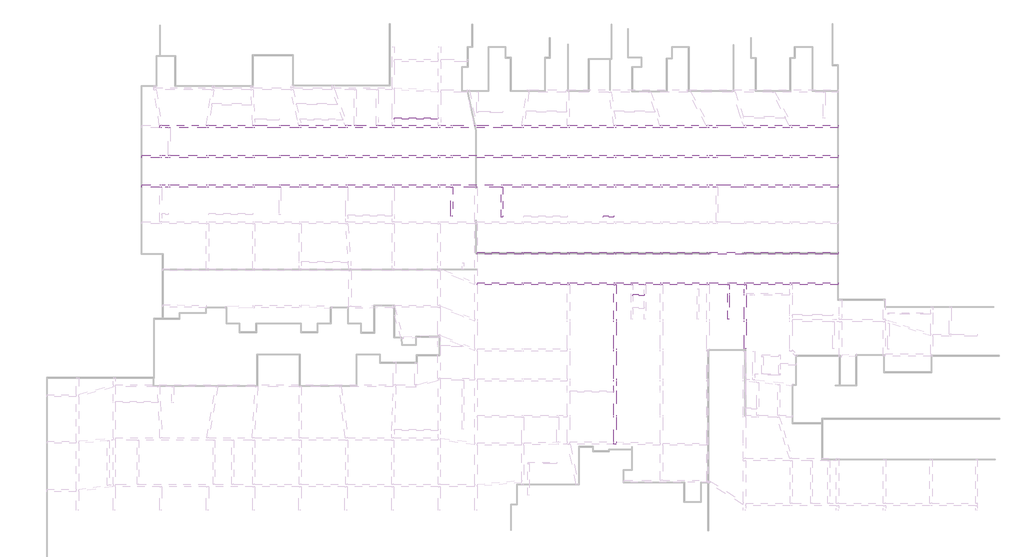
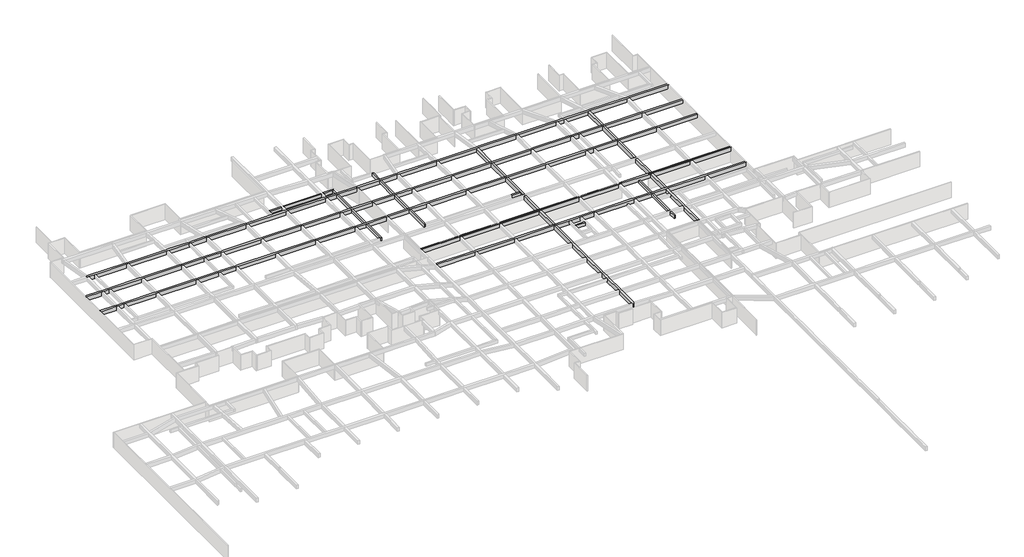
# One storey, part 15 of 16: 13 beams.
"""IFC4 building model written with IfcOpenShell, lengths in millimetres."""

from ifc_helpers import new_model, si_unit, frame, origin, place, context, project, spatial, polyline, outline, extrude, faceted_brep, element, save

model = new_model("IFC4")

# Units and contexts
model_context = context("Model", 3, world=origin())
ifc_project = project(units=[si_unit("LENGTHUNIT", "METRE", prefix="MILLI")], contexts=[model_context])

# Site, building, storey
site = spatial("IfcSite", under=ifc_project)
building = spatial("IfcBuilding", under=site)
storey = spatial("IfcBuildingStorey", under=building, Name="户型图", Elevation=0.0)

# Beams
placement = place(None, origin())
element("IfcBeam", 1, ObjectType="混凝土 - 矩形梁 : KL_beam", at=placement, inside=storey, context=model_context, shape_type="Brep", body=[
    faceted_brep([(204626.3581141, 190295.7397162, 3300.0), (204626.3581141, 189895.7397162, 3300.0), (204626.3581141, 189895.7397162, 2500.0), (204626.3581141, 190295.7397162, 2500.0), (196548.907663, 190295.7397162, 3300.0), (196099.6244537, 190295.7397162, 3300.0), (188560.8339464, 190295.7397162, 3300.0), (188139.6298053, 190295.7397162, 3300.0), (183653.5662503, 190295.7397162, 3300.0), (183353.5662503, 190295.7397162, 3300.0), (182035.6002826, 190295.7397162, 3300.0), (181581.1727256, 190295.7397162, 3300.0), (173958.7712722, 190295.7397162, 3300.0), (173535.6280152, 190295.7397162, 3300.0), (165889.741752, 190295.7397162, 3300.0), (165485.7043374, 190295.7397162, 3300.0), (157809.3486586, 190295.7397162, 3300.0), (157409.1048409, 190295.7397162, 3300.0), (149847.7648646, 190295.7397162, 3300.0), (149443.4649924, 190295.7397162, 3300.0), (146146.1090193, 190295.7397162, 3300.0), (145846.1090193, 190295.7397162, 3300.0), (141582.1467117, 190295.7397162, 3300.0), (141173.2104737, 190295.7397162, 3300.0), (137401.0841862, 190295.7397162, 3300.0), (137101.0841862, 190295.7397162, 3300.0), (135274.2374796, 190295.7397162, 3300.0), (134874.2374796, 190295.7397162, 3300.0), (127216.2109037, 190295.7397162, 3300.0), (126816.2109037, 190295.7397162, 3300.0), (124373.9303911, 190295.7397162, 3300.0), (124073.9303911, 190295.7397162, 3300.0), (120573.9609037, 190295.7397162, 3300.0), (120273.9609037, 190295.7397162, 3300.0), (119056.2524113, 190295.7397162, 3300.0), (118630.5813023, 190295.7397162, 3300.0), (110975.298087, 190295.7397162, 3300.0), (110564.7764439, 190295.7397162, 3300.0), (107420.783903, 190295.7397162, 3300.0), (107120.783903, 190295.7397162, 3300.0), (102906.003817, 190295.7397162, 3300.0), (102505.4548786, 190295.7397162, 3300.0), (94846.2845851, 190295.7397162, 3300.0), (94442.3535561, 190295.7397162, 3300.0), (86664.9777116, 190295.7397162, 3300.0), (86294.1615746, 190295.7397162, 3300.0), (86294.1615746, 189895.7397162, 3300.0), (86694.1615746, 189895.7397162, 3300.0), (87820.783903, 189895.7397162, 3300.0), (88120.783903, 189895.7397162, 3300.0), (94416.2109037, 189895.7397162, 3300.0), (94816.2109037, 189895.7397162, 3300.0), (102516.2109037, 189895.7397162, 3300.0), (102916.2109037, 189895.7397162, 3300.0), (107120.783903, 189895.7397162, 3300.0), (107420.783903, 189895.7397162, 3300.0), (110616.2109037, 189895.7397162, 3300.0), (111016.2109037, 189895.7397162, 3300.0), (118716.2109037, 189895.7397162, 3300.0), (119116.2109037, 189895.7397162, 3300.0), (126816.2109037, 189895.7397162, 3300.0), (127216.2109037, 189895.7397162, 3300.0), (134816.2109037, 189895.7397162, 3300.0), (135216.2109037, 189895.7397162, 3300.0), (137101.0841862, 189895.7397162, 3300.0), (137401.0841862, 189895.7397162, 3300.0), (145846.1090193, 189895.7397162, 3300.0), (146146.1090193, 189895.7397162, 3300.0), (149416.2109037, 189895.7397162, 3300.0), (149816.2109037, 189895.7397162, 3300.0), (157416.2109037, 189895.7397162, 3300.0), (157816.2109037, 189895.7397162, 3300.0), (165516.2109037, 189895.7397162, 3300.0), (165916.2109037, 189895.7397162, 3300.0), (173616.2109037, 189895.7397162, 3300.0), (174016.2109037, 189895.7397162, 3300.0), (181716.2109037, 189895.7397162, 3300.0), (182116.2109037, 189895.7397162, 3300.0), (183353.5662503, 189895.7397162, 3300.0), (183653.5662503, 189895.7397162, 3300.0), (188216.2109037, 189895.7397162, 3300.0), (188616.2109037, 189895.7397162, 3300.0), (196226.5590225, 189895.7397162, 3300.0), (196626.5590225, 189895.7397162, 3300.0), (86294.1615746, 189895.7397162, 2500.0), (86694.1615746, 189895.7397162, 2500.0), (94416.2109037, 189895.7397162, 2500.0), (94816.2109037, 189895.7397162, 2500.0), (102516.2109037, 189895.7397162, 2500.0), (102916.2109037, 189895.7397162, 2500.0), (110616.2109037, 189895.7397162, 2500.0), (111016.2109037, 189895.7397162, 2500.0), (118716.2109037, 189895.7397162, 2500.0), (119116.2109037, 189895.7397162, 2500.0), (126816.2109037, 189895.7397162, 2500.0), (127216.2109037, 189895.7397162, 2500.0), (134816.2109037, 189895.7397162, 2500.0), (135216.2109037, 189895.7397162, 2500.0), (149416.2109037, 189895.7397162, 2500.0), (149816.2109037, 189895.7397162, 2500.0), (157416.2109037, 189895.7397162, 2500.0), (157816.2109037, 189895.7397162, 2500.0), (165516.2109037, 189895.7397162, 2500.0), (165916.2109037, 189895.7397162, 2500.0), (173616.2109037, 189895.7397162, 2500.0), (174016.2109037, 189895.7397162, 2500.0), (181716.2109037, 189895.7397162, 2500.0), (182116.2109037, 189895.7397162, 2500.0), (188216.2109037, 189895.7397162, 2500.0), (188616.2109037, 189895.7397162, 2500.0), (196226.5590225, 189895.7397162, 2500.0), (196626.5590225, 189895.7397162, 2500.0), (86294.1615746, 190295.7397162, 2500.0), (86664.9777116, 190295.7397162, 2500.0), (94442.3535561, 190295.7397162, 2500.0), (94846.2845851, 190295.7397162, 2500.0), (102505.4548786, 190295.7397162, 2500.0), (102906.003817, 190295.7397162, 2500.0), (110564.7764439, 190295.7397162, 2500.0), (110975.298087, 190295.7397162, 2500.0), (118630.5813023, 190295.7397162, 2500.0), (119056.2524113, 190295.7397162, 2500.0), (126816.2109037, 190295.7397162, 2500.0), (127216.2109037, 190295.7397162, 2500.0), (134874.2374796, 190295.7397162, 2500.0), (135274.2374796, 190295.7397162, 2500.0), (141173.2104737, 190295.7397162, 2500.0), (141582.1467117, 190295.7397162, 2500.0), (149443.4649924, 190295.7397162, 2500.0), (149847.7648646, 190295.7397162, 2500.0), (157409.1048409, 190295.7397162, 2500.0), (157809.3486586, 190295.7397162, 2500.0), (165485.7043374, 190295.7397162, 2500.0), (165889.741752, 190295.7397162, 2500.0), (173535.6280152, 190295.7397162, 2500.0), (173958.7712722, 190295.7397162, 2500.0), (181581.1727256, 190295.7397162, 2500.0), (182035.6002826, 190295.7397162, 2500.0), (188139.6298053, 190295.7397162, 2500.0), (188560.8339464, 190295.7397162, 2500.0), (196099.6244537, 190295.7397162, 2500.0), (196548.907663, 190295.7397162, 2500.0)], [[[0, 1, 2, 3]], [[1, 0, 4, 5, 6, 7, 8, 9, 10, 11, 12, 13, 14, 15, 16, 17, 18, 19, 20, 21, 22, 23, 24, 25, 26, 27, 28, 29, 30, 31, 32, 33, 34, 35, 36, 37, 38, 39, 40, 41, 42, 43, 44, 45, 46, 47, 48, 49, 50, 51, 52, 53, 54, 55, 56, 57, 58, 59, 60, 61, 62, 63, 64, 65, 66, 67, 68, 69, 70, 71, 72, 73, 74, 75, 76, 77, 78, 79, 80, 81, 82, 83]], [[2, 1, 83, 82, 81, 80, 79, 78, 77, 76, 75, 74, 73, 72, 71, 70, 69, 68, 67, 66, 65, 64, 63, 62, 61, 60, 59, 58, 57, 56, 55, 54, 53, 52, 51, 50, 49, 48, 47, 46, 84, 85, 86, 87, 88, 89, 90, 91, 92, 93, 94, 95, 96, 97, 98, 99, 100, 101, 102, 103, 104, 105, 106, 107, 108, 109, 110, 111]], [[3, 2, 111, 110, 109, 108, 107, 106, 105, 104, 103, 102, 101, 100, 99, 98, 97, 96, 95, 94, 93, 92, 91, 90, 89, 88, 87, 86, 85, 84, 112, 113, 114, 115, 116, 117, 118, 119, 120, 121, 122, 123, 124, 125, 126, 127, 128, 129, 130, 131, 132, 133, 134, 135, 136, 137, 138, 139, 140, 141]], [[0, 3, 141, 140, 139, 138, 137, 136, 135, 134, 133, 132, 131, 130, 129, 128, 127, 126, 125, 124, 123, 122, 121, 120, 119, 118, 117, 116, 115, 114, 113, 112, 45, 44, 43, 42, 41, 40, 39, 38, 37, 36, 35, 34, 33, 32, 31, 30, 29, 28, 27, 26, 25, 24, 23, 22, 21, 20, 19, 18, 17, 16, 15, 14, 13, 12, 11, 10, 9, 8, 7, 6, 5, 4]], [[46, 45, 112, 84]]]),
])
element("IfcBeam", 2, ObjectType="混凝土 - 矩形梁 : KL_beam", at=placement, inside=storey, context=model_context, shape_type="Brep", body=[
    faceted_brep([(204626.2466536, 185072.5884701, 3300.0), (204626.2466536, 184672.5884701, 3300.0), (204626.2466536, 184672.5884701, 2500.0), (204626.2466536, 185072.5884701, 2500.0), (83129.2466536, 185072.5884701, 3300.0), (83129.2466536, 185072.5884701, 2500.0), (83129.2466536, 184672.5884701, 2500.0), (83129.2466536, 184672.5884701, 3300.0), (196626.5590225, 185072.5884701, 3300.0), (196226.5590225, 185072.5884701, 3300.0), (188616.2109037, 185072.5884701, 3300.0), (188216.2109037, 185072.5884701, 3300.0), (183653.5662503, 185072.5884701, 3300.0), (183353.5662503, 185072.5884701, 3300.0), (182116.2109037, 185072.5884701, 3300.0), (181716.2109037, 185072.5884701, 3300.0), (174016.2109037, 185072.5884701, 3300.0), (173616.2109037, 185072.5884701, 3300.0), (165916.2109037, 185072.5884701, 3300.0), (165516.2109037, 185072.5884701, 3300.0), (157816.2109037, 185072.5884701, 3300.0), (157416.2109037, 185072.5884701, 3300.0), (149816.2109037, 185072.5884701, 3300.0), (149416.2109037, 185072.5884701, 3300.0), (146146.1090193, 185072.5884701, 3300.0), (145846.1090193, 185072.5884701, 3300.0), (137401.0841862, 185072.5884701, 3300.0), (137101.0841862, 185072.5884701, 3300.0), (135216.2109037, 185072.5884701, 3300.0), (134816.2109037, 185072.5884701, 3300.0), (127216.2109037, 185072.5884701, 3300.0), (126816.2109037, 185072.5884701, 3300.0), (119116.2109037, 185072.5884701, 3300.0), (118716.2109037, 185072.5884701, 3300.0), (111016.2109037, 185072.5884701, 3300.0), (110616.2109037, 185072.5884701, 3300.0), (107420.783903, 185072.5884701, 3300.0), (107120.783903, 185072.5884701, 3300.0), (102916.2109037, 185072.5884701, 3300.0), (102516.2109037, 185072.5884701, 3300.0), (94816.2109037, 185072.5884701, 3300.0), (94416.2109037, 185072.5884701, 3300.0), (88120.783903, 185072.5884701, 3300.0), (87820.783903, 185072.5884701, 3300.0), (86694.1615746, 185072.5884701, 3300.0), (86294.1615746, 185072.5884701, 3300.0), (86294.1615746, 184672.5884701, 3300.0), (86694.1615746, 184672.5884701, 3300.0), (87820.783903, 184672.5884701, 3300.0), (88120.783903, 184672.5884701, 3300.0), (94416.2109037, 184672.5884701, 3300.0), (94816.2109037, 184672.5884701, 3300.0), (102516.2109037, 184672.5884701, 3300.0), (102916.2109037, 184672.5884701, 3300.0), (107120.783903, 184672.5884701, 3300.0), (107420.783903, 184672.5884701, 3300.0), (110616.2109037, 184672.5884701, 3300.0), (111016.2109037, 184672.5884701, 3300.0), (118716.2109037, 184672.5884701, 3300.0), (119116.2109037, 184672.5884701, 3300.0), (126816.2109037, 184672.5884701, 3300.0), (127216.2109037, 184672.5884701, 3300.0), (134816.2109037, 184672.5884701, 3300.0), (135216.2109037, 184672.5884701, 3300.0), (137101.0841862, 184672.5884701, 3300.0), (137401.0841862, 184672.5884701, 3300.0), (145846.1090193, 184672.5884701, 3300.0), (146146.1090193, 184672.5884701, 3300.0), (149416.2109037, 184672.5884701, 3300.0), (149816.2109037, 184672.5884701, 3300.0), (157416.2109037, 184672.5884701, 3300.0), (157816.2109037, 184672.5884701, 3300.0), (165516.2109037, 184672.5884701, 3300.0), (165916.2109037, 184672.5884701, 3300.0), (173616.2109037, 184672.5884701, 3300.0), (174016.2109037, 184672.5884701, 3300.0), (181716.2109037, 184672.5884701, 3300.0), (182116.2109037, 184672.5884701, 3300.0), (183353.5662503, 184672.5884701, 3300.0), (183653.5662503, 184672.5884701, 3300.0), (188216.2109037, 184672.5884701, 3300.0), (188616.2109037, 184672.5884701, 3300.0), (196226.5590225, 184672.5884701, 3300.0), (196626.5590225, 184672.5884701, 3300.0), (86294.1615746, 184672.5884701, 2500.0), (86694.1615746, 184672.5884701, 2500.0), (94416.2109037, 184672.5884701, 2500.0), (94816.2109037, 184672.5884701, 2500.0), (102516.2109037, 184672.5884701, 2500.0), (102916.2109037, 184672.5884701, 2500.0), (110616.2109037, 184672.5884701, 2500.0), (111016.2109037, 184672.5884701, 2500.0), (118716.2109037, 184672.5884701, 2500.0), (119116.2109037, 184672.5884701, 2500.0), (126816.2109037, 184672.5884701, 2500.0), (127216.2109037, 184672.5884701, 2500.0), (134816.2109037, 184672.5884701, 2500.0), (135216.2109037, 184672.5884701, 2500.0), (149416.2109037, 184672.5884701, 2500.0), (149816.2109037, 184672.5884701, 2500.0), (157416.2109037, 184672.5884701, 2500.0), (157816.2109037, 184672.5884701, 2500.0), (165516.2109037, 184672.5884701, 2500.0), (165916.2109037, 184672.5884701, 2500.0), (173616.2109037, 184672.5884701, 2500.0), (174016.2109037, 184672.5884701, 2500.0), (181716.2109037, 184672.5884701, 2500.0), (182116.2109037, 184672.5884701, 2500.0), (188216.2109037, 184672.5884701, 2500.0), (188616.2109037, 184672.5884701, 2500.0), (196226.5590225, 184672.5884701, 2500.0), (196626.5590225, 184672.5884701, 2500.0), (86294.1615746, 185072.5884701, 2500.0), (86694.1615746, 185072.5884701, 2500.0), (94416.2109037, 185072.5884701, 2500.0), (94816.2109037, 185072.5884701, 2500.0), (102516.2109037, 185072.5884701, 2500.0), (102916.2109037, 185072.5884701, 2500.0), (110616.2109037, 185072.5884701, 2500.0), (111016.2109037, 185072.5884701, 2500.0), (118716.2109037, 185072.5884701, 2500.0), (119116.2109037, 185072.5884701, 2500.0), (126816.2109037, 185072.5884701, 2500.0), (127216.2109037, 185072.5884701, 2500.0), (134816.2109037, 185072.5884701, 2500.0), (135216.2109037, 185072.5884701, 2500.0), (149416.2109037, 185072.5884701, 2500.0), (149816.2109037, 185072.5884701, 2500.0), (157416.2109037, 185072.5884701, 2500.0), (157816.2109037, 185072.5884701, 2500.0), (165516.2109037, 185072.5884701, 2500.0), (165916.2109037, 185072.5884701, 2500.0), (173616.2109037, 185072.5884701, 2500.0), (174016.2109037, 185072.5884701, 2500.0), (181716.2109037, 185072.5884701, 2500.0), (182116.2109037, 185072.5884701, 2500.0), (188216.2109037, 185072.5884701, 2500.0), (188616.2109037, 185072.5884701, 2500.0), (196226.5590225, 185072.5884701, 2500.0), (196626.5590225, 185072.5884701, 2500.0)], [[[0, 1, 2, 3]], [[4, 5, 6, 7]], [[1, 0, 8, 9, 10, 11, 12, 13, 14, 15, 16, 17, 18, 19, 20, 21, 22, 23, 24, 25, 26, 27, 28, 29, 30, 31, 32, 33, 34, 35, 36, 37, 38, 39, 40, 41, 42, 43, 44, 45, 4, 7, 46, 47, 48, 49, 50, 51, 52, 53, 54, 55, 56, 57, 58, 59, 60, 61, 62, 63, 64, 65, 66, 67, 68, 69, 70, 71, 72, 73, 74, 75, 76, 77, 78, 79, 80, 81, 82, 83]], [[2, 1, 83, 82, 81, 80, 79, 78, 77, 76, 75, 74, 73, 72, 71, 70, 69, 68, 67, 66, 65, 64, 63, 62, 61, 60, 59, 58, 57, 56, 55, 54, 53, 52, 51, 50, 49, 48, 47, 46, 7, 6, 84, 85, 86, 87, 88, 89, 90, 91, 92, 93, 94, 95, 96, 97, 98, 99, 100, 101, 102, 103, 104, 105, 106, 107, 108, 109, 110, 111]], [[3, 2, 111, 110, 109, 108, 107, 106, 105, 104, 103, 102, 101, 100, 99, 98, 97, 96, 95, 94, 93, 92, 91, 90, 89, 88, 87, 86, 85, 84, 6, 5, 112, 113, 114, 115, 116, 117, 118, 119, 120, 121, 122, 123, 124, 125, 126, 127, 128, 129, 130, 131, 132, 133, 134, 135, 136, 137, 138, 139]], [[0, 3, 139, 138, 137, 136, 135, 134, 133, 132, 131, 130, 129, 128, 127, 126, 125, 124, 123, 122, 121, 120, 119, 118, 117, 116, 115, 114, 113, 112, 5, 4, 45, 44, 43, 42, 41, 40, 39, 38, 37, 36, 35, 34, 33, 32, 31, 30, 29, 28, 27, 26, 25, 24, 23, 22, 21, 20, 19, 18, 17, 16, 15, 14, 13, 12, 11, 10, 9, 8]]]),
])
element("IfcBeam", 3, ObjectType="混凝土 - 矩形梁 : KL_beam", at=placement, inside=storey, context=model_context, shape_type="Brep", body=[
    faceted_brep([(204626.2466536, 179912.5884701, 3300.0), (204626.2466536, 179512.5884701, 3300.0), (204626.2466536, 179512.5884701, 2500.0), (204626.2466536, 179912.5884701, 2500.0), (83129.2466536, 179912.5884701, 3300.0), (83129.2466536, 179912.5884701, 2500.0), (83129.2466536, 179512.5884701, 2500.0), (83129.2466536, 179512.5884701, 3300.0), (196626.5590225, 179912.5884701, 3300.0), (196226.5590225, 179912.5884701, 3300.0), (188616.2109037, 179912.5884701, 3300.0), (188216.2109037, 179912.5884701, 3300.0), (183653.5662503, 179912.5884701, 3300.0), (183353.5662503, 179912.5884701, 3300.0), (182116.2109037, 179912.5884701, 3300.0), (181716.2109037, 179912.5884701, 3300.0), (174016.2109037, 179912.5884701, 3300.0), (173616.2109037, 179912.5884701, 3300.0), (165916.2109037, 179912.5884701, 3300.0), (165516.2109037, 179912.5884701, 3300.0), (157816.2109037, 179912.5884701, 3300.0), (157416.2109037, 179912.5884701, 3300.0), (149816.2109037, 179912.5884701, 3300.0), (149416.2109037, 179912.5884701, 3300.0), (146146.1090193, 179912.5884701, 3300.0), (145846.1090193, 179912.5884701, 3300.0), (137401.0841862, 179912.5884701, 3300.0), (137101.0841862, 179912.5884701, 3300.0), (135216.2109037, 179912.5884701, 3300.0), (134816.2109037, 179912.5884701, 3300.0), (127216.2109037, 179912.5884701, 3300.0), (126816.2109037, 179912.5884701, 3300.0), (119116.2109037, 179912.5884701, 3300.0), (118716.2109037, 179912.5884701, 3300.0), (111016.2109037, 179912.5884701, 3300.0), (110616.2109037, 179912.5884701, 3300.0), (107420.783903, 179912.5884701, 3300.0), (107120.783903, 179912.5884701, 3300.0), (102916.2109037, 179912.5884701, 3300.0), (102516.2109037, 179912.5884701, 3300.0), (94816.2109037, 179912.5884701, 3300.0), (94416.2109037, 179912.5884701, 3300.0), (88120.783903, 179912.5884701, 3300.0), (87820.783903, 179912.5884701, 3300.0), (86694.1615746, 179912.5884701, 3300.0), (86294.1615746, 179912.5884701, 3300.0), (86294.1615746, 179512.5884701, 3300.0), (86694.1615746, 179512.5884701, 3300.0), (87820.783903, 179512.5884701, 3300.0), (88120.783903, 179512.5884701, 3300.0), (94416.2109037, 179512.5884701, 3300.0), (94816.2109037, 179512.5884701, 3300.0), (102516.2109037, 179512.5884701, 3300.0), (102916.2109037, 179512.5884701, 3300.0), (107120.783903, 179512.5884701, 3300.0), (107420.783903, 179512.5884701, 3300.0), (110616.2109037, 179512.5884701, 3300.0), (111016.2109037, 179512.5884701, 3300.0), (118716.2109037, 179512.5884701, 3300.0), (119116.2109037, 179512.5884701, 3300.0), (126816.2109037, 179512.5884701, 3300.0), (127216.2109037, 179512.5884701, 3300.0), (134816.2109037, 179512.5884701, 3300.0), (135216.2109037, 179512.5884701, 3300.0), (137101.0841862, 179512.5884701, 3300.0), (137401.0841862, 179512.5884701, 3300.0), (141260.1899051, 179512.5884701, 3300.0), (141660.1899051, 179512.5884701, 3300.0), (145846.1090193, 179512.5884701, 3300.0), (146146.1090193, 179512.5884701, 3300.0), (149416.2109037, 179512.5884701, 3300.0), (149816.2109037, 179512.5884701, 3300.0), (157416.2109037, 179512.5884701, 3300.0), (157816.2109037, 179512.5884701, 3300.0), (165516.2109037, 179512.5884701, 3300.0), (165916.2109037, 179512.5884701, 3300.0), (173616.2109037, 179512.5884701, 3300.0), (174016.2109037, 179512.5884701, 3300.0), (181716.2109037, 179512.5884701, 3300.0), (182116.2109037, 179512.5884701, 3300.0), (183353.5662503, 179512.5884701, 3300.0), (183653.5662503, 179512.5884701, 3300.0), (188216.2109037, 179512.5884701, 3300.0), (188616.2109037, 179512.5884701, 3300.0), (196226.5590225, 179512.5884701, 3300.0), (196626.5590225, 179512.5884701, 3300.0), (86294.1615746, 179512.5884701, 2500.0), (86694.1615746, 179512.5884701, 2500.0), (94416.2109037, 179512.5884701, 2500.0), (94816.2109037, 179512.5884701, 2500.0), (102516.2109037, 179512.5884701, 2500.0), (102916.2109037, 179512.5884701, 2500.0), (110616.2109037, 179512.5884701, 2500.0), (111016.2109037, 179512.5884701, 2500.0), (118716.2109037, 179512.5884701, 2500.0), (119116.2109037, 179512.5884701, 2500.0), (126816.2109037, 179512.5884701, 2500.0), (127216.2109037, 179512.5884701, 2500.0), (134816.2109037, 179512.5884701, 2500.0), (135216.2109037, 179512.5884701, 2500.0), (141260.1899051, 179512.5884701, 2500.0), (141660.1899051, 179512.5884701, 2500.0), (149416.2109037, 179512.5884701, 2500.0), (149816.2109037, 179512.5884701, 2500.0), (157416.2109037, 179512.5884701, 2500.0), (157816.2109037, 179512.5884701, 2500.0), (165516.2109037, 179512.5884701, 2500.0), (165916.2109037, 179512.5884701, 2500.0), (173616.2109037, 179512.5884701, 2500.0), (174016.2109037, 179512.5884701, 2500.0), (181716.2109037, 179512.5884701, 2500.0), (182116.2109037, 179512.5884701, 2500.0), (188216.2109037, 179512.5884701, 2500.0), (188616.2109037, 179512.5884701, 2500.0), (196226.5590225, 179512.5884701, 2500.0), (196626.5590225, 179512.5884701, 2500.0), (86294.1615746, 179912.5884701, 2500.0), (86694.1615746, 179912.5884701, 2500.0), (94416.2109037, 179912.5884701, 2500.0), (94816.2109037, 179912.5884701, 2500.0), (102516.2109037, 179912.5884701, 2500.0), (102916.2109037, 179912.5884701, 2500.0), (110616.2109037, 179912.5884701, 2500.0), (111016.2109037, 179912.5884701, 2500.0), (118716.2109037, 179912.5884701, 2500.0), (119116.2109037, 179912.5884701, 2500.0), (126816.2109037, 179912.5884701, 2500.0), (127216.2109037, 179912.5884701, 2500.0), (134816.2109037, 179912.5884701, 2500.0), (135216.2109037, 179912.5884701, 2500.0), (149416.2109037, 179912.5884701, 2500.0), (149816.2109037, 179912.5884701, 2500.0), (157416.2109037, 179912.5884701, 2500.0), (157816.2109037, 179912.5884701, 2500.0), (165516.2109037, 179912.5884701, 2500.0), (165916.2109037, 179912.5884701, 2500.0), (173616.2109037, 179912.5884701, 2500.0), (174016.2109037, 179912.5884701, 2500.0), (181716.2109037, 179912.5884701, 2500.0), (182116.2109037, 179912.5884701, 2500.0), (188216.2109037, 179912.5884701, 2500.0), (188616.2109037, 179912.5884701, 2500.0), (196226.5590225, 179912.5884701, 2500.0), (196626.5590225, 179912.5884701, 2500.0)], [[[0, 1, 2, 3]], [[4, 5, 6, 7]], [[1, 0, 8, 9, 10, 11, 12, 13, 14, 15, 16, 17, 18, 19, 20, 21, 22, 23, 24, 25, 26, 27, 28, 29, 30, 31, 32, 33, 34, 35, 36, 37, 38, 39, 40, 41, 42, 43, 44, 45, 4, 7, 46, 47, 48, 49, 50, 51, 52, 53, 54, 55, 56, 57, 58, 59, 60, 61, 62, 63, 64, 65, 66, 67, 68, 69, 70, 71, 72, 73, 74, 75, 76, 77, 78, 79, 80, 81, 82, 83, 84, 85]], [[2, 1, 85, 84, 83, 82, 81, 80, 79, 78, 77, 76, 75, 74, 73, 72, 71, 70, 69, 68, 67, 66, 65, 64, 63, 62, 61, 60, 59, 58, 57, 56, 55, 54, 53, 52, 51, 50, 49, 48, 47, 46, 7, 6, 86, 87, 88, 89, 90, 91, 92, 93, 94, 95, 96, 97, 98, 99, 100, 101, 102, 103, 104, 105, 106, 107, 108, 109, 110, 111, 112, 113, 114, 115]], [[3, 2, 115, 114, 113, 112, 111, 110, 109, 108, 107, 106, 105, 104, 103, 102, 101, 100, 99, 98, 97, 96, 95, 94, 93, 92, 91, 90, 89, 88, 87, 86, 6, 5, 116, 117, 118, 119, 120, 121, 122, 123, 124, 125, 126, 127, 128, 129, 130, 131, 132, 133, 134, 135, 136, 137, 138, 139, 140, 141, 142, 143]], [[0, 3, 143, 142, 141, 140, 139, 138, 137, 136, 135, 134, 133, 132, 131, 130, 129, 128, 127, 126, 125, 124, 123, 122, 121, 120, 119, 118, 117, 116, 5, 4, 45, 44, 43, 42, 41, 40, 39, 38, 37, 36, 35, 34, 33, 32, 31, 30, 29, 28, 27, 26, 25, 24, 23, 22, 21, 20, 19, 18, 17, 16, 15, 14, 13, 12, 11, 10, 9, 8]]]),
])
element("IfcBeam", 4, ObjectType="混凝土 - 矩形梁 : KL_beam", at=placement, inside=storey, context=model_context, shape_type="Brep", body=[
    faceted_brep([(204626.3818873, 162847.0169772, 3300.0), (204626.3818873, 162447.0169772, 3300.0), (204626.3818873, 162447.0169772, 2500.0), (204626.3818873, 162847.0169772, 2500.0), (196626.5590225, 162847.0169772, 3300.0), (196226.5590225, 162847.0169772, 3300.0), (188616.2109037, 162847.0169772, 3300.0), (188216.2109037, 162847.0169772, 3300.0), (185653.3391382, 162847.0169772, 3300.0), (185353.3391382, 162847.0169772, 3300.0), (182116.2109037, 162847.0169772, 3300.0), (181716.2109037, 162847.0169772, 3300.0), (174016.2109037, 162847.0169772, 3300.0), (173616.2109037, 162847.0169772, 3300.0), (165916.2109037, 162847.0169772, 3300.0), (165516.2109037, 162847.0169772, 3300.0), (157816.2109037, 162847.0169772, 3300.0), (157416.2109037, 162847.0169772, 3300.0), (149816.2109037, 162847.0169772, 3300.0), (149416.2109037, 162847.0169772, 3300.0), (141666.2091209, 162847.0169772, 3300.0), (141666.2091209, 162447.0169772, 3300.0), (149416.2109037, 162447.0169772, 3300.0), (149816.2109037, 162447.0169772, 3300.0), (157416.2109037, 162447.0169772, 3300.0), (157816.2109037, 162447.0169772, 3300.0), (165516.2109037, 162447.0169772, 3300.0), (165916.2109037, 162447.0169772, 3300.0), (168541.2109037, 162447.0169772, 3300.0), (168841.2109037, 162447.0169772, 3300.0), (170791.2109037, 162447.0169772, 3300.0), (171091.2109037, 162447.0169772, 3300.0), (173616.2109037, 162447.0169772, 3300.0), (174016.2109037, 162447.0169772, 3300.0), (181716.2109037, 162447.0169772, 3300.0), (182116.2109037, 162447.0169772, 3300.0), (185353.3391382, 162447.0169772, 3300.0), (185653.3391382, 162447.0169772, 3300.0), (188216.2109037, 162447.0169772, 3300.0), (188616.2109037, 162447.0169772, 3300.0), (196226.5590225, 162447.0169772, 3300.0), (196626.5590225, 162447.0169772, 3300.0), (141666.2091209, 162447.0169772, 2500.0), (149416.2109037, 162447.0169772, 2500.0), (149816.2109037, 162447.0169772, 2500.0), (157416.2109037, 162447.0169772, 2500.0), (157816.2109037, 162447.0169772, 2500.0), (165516.2109037, 162447.0169772, 2500.0), (165916.2109037, 162447.0169772, 2500.0), (173616.2109037, 162447.0169772, 2500.0), (174016.2109037, 162447.0169772, 2500.0), (181716.2109037, 162447.0169772, 2500.0), (182116.2109037, 162447.0169772, 2500.0), (188216.2109037, 162447.0169772, 2500.0), (188616.2109037, 162447.0169772, 2500.0), (196226.5590225, 162447.0169772, 2500.0), (196626.5590225, 162447.0169772, 2500.0), (141666.2091209, 162847.0169772, 2500.0), (149416.2109037, 162847.0169772, 2500.0), (149816.2109037, 162847.0169772, 2500.0), (157416.2109037, 162847.0169772, 2500.0), (157816.2109037, 162847.0169772, 2500.0), (165516.2109037, 162847.0169772, 2500.0), (165916.2109037, 162847.0169772, 2500.0), (173616.2109037, 162847.0169772, 2500.0), (174016.2109037, 162847.0169772, 2500.0), (181716.2109037, 162847.0169772, 2500.0), (182116.2109037, 162847.0169772, 2500.0), (188216.2109037, 162847.0169772, 2500.0), (188616.2109037, 162847.0169772, 2500.0), (196226.5590225, 162847.0169772, 2500.0), (196626.5590225, 162847.0169772, 2500.0)], [[[0, 1, 2, 3]], [[1, 0, 4, 5, 6, 7, 8, 9, 10, 11, 12, 13, 14, 15, 16, 17, 18, 19, 20, 21, 22, 23, 24, 25, 26, 27, 28, 29, 30, 31, 32, 33, 34, 35, 36, 37, 38, 39, 40, 41]], [[2, 1, 41, 40, 39, 38, 37, 36, 35, 34, 33, 32, 31, 30, 29, 28, 27, 26, 25, 24, 23, 22, 21, 42, 43, 44, 45, 46, 47, 48, 49, 50, 51, 52, 53, 54, 55, 56]], [[3, 2, 56, 55, 54, 53, 52, 51, 50, 49, 48, 47, 46, 45, 44, 43, 42, 57, 58, 59, 60, 61, 62, 63, 64, 65, 66, 67, 68, 69, 70, 71]], [[0, 3, 71, 70, 69, 68, 67, 66, 65, 64, 63, 62, 61, 60, 59, 58, 57, 20, 19, 18, 17, 16, 15, 14, 13, 12, 11, 10, 9, 8, 7, 6, 5, 4]], [[20, 57, 42, 21]]]),
])
element("IfcBeam", 5, ObjectType="混凝土 - 矩形梁 : KL_beam", at=placement, inside=storey, context=model_context, shape_type="Brep", body=[
    faceted_brep([(204626.3818873, 168162.578939, 3300.0), (204626.3818873, 167762.578939, 3300.0), (204626.3818873, 167762.578939, 2500.0), (204626.3818873, 168162.578939, 2500.0), (196626.5590225, 168162.578939, 3300.0), (196226.5590225, 168162.578939, 3300.0), (188616.2109037, 168162.578939, 3300.0), (188216.2109037, 168162.578939, 3300.0), (182116.2109037, 168162.578939, 3300.0), (181716.2109037, 168162.578939, 3300.0), (174016.2109037, 168162.578939, 3300.0), (173616.2109037, 168162.578939, 3300.0), (165916.2109037, 168162.578939, 3300.0), (165516.2109037, 168162.578939, 3300.0), (157816.2109037, 168162.578939, 3300.0), (157416.2109037, 168162.578939, 3300.0), (149816.2109037, 168162.578939, 3300.0), (149416.2109037, 168162.578939, 3300.0), (141666.2091209, 168162.578939, 3300.0), (141666.2091209, 167762.578939, 3300.0), (149416.2109037, 167762.578939, 3300.0), (149816.2109037, 167762.578939, 3300.0), (157416.2109037, 167762.578939, 3300.0), (157816.2109037, 167762.578939, 3300.0), (165516.2109037, 167762.578939, 3300.0), (165916.2109037, 167762.578939, 3300.0), (173616.2109037, 167762.578939, 3300.0), (174016.2109037, 167762.578939, 3300.0), (181716.2109037, 167762.578939, 3300.0), (182116.2109037, 167762.578939, 3300.0), (188216.2109037, 167762.578939, 3300.0), (188616.2109037, 167762.578939, 3300.0), (196226.5590225, 167762.578939, 3300.0), (196626.5590225, 167762.578939, 3300.0), (141666.2091209, 167762.578939, 2500.0), (149416.2109037, 167762.578939, 2500.0), (149816.2109037, 167762.578939, 2500.0), (157416.2109037, 167762.578939, 2500.0), (157816.2109037, 167762.578939, 2500.0), (165516.2109037, 167762.578939, 2500.0), (165916.2109037, 167762.578939, 2500.0), (173616.2109037, 167762.578939, 2500.0), (174016.2109037, 167762.578939, 2500.0), (181716.2109037, 167762.578939, 2500.0), (182116.2109037, 167762.578939, 2500.0), (188216.2109037, 167762.578939, 2500.0), (188616.2109037, 167762.578939, 2500.0), (196226.5590225, 167762.578939, 2500.0), (196626.5590225, 167762.578939, 2500.0), (141666.2091209, 168162.578939, 2500.0), (149416.2109037, 168162.578939, 2500.0), (149816.2109037, 168162.578939, 2500.0), (157416.2109037, 168162.578939, 2500.0), (157816.2109037, 168162.578939, 2500.0), (165516.2109037, 168162.578939, 2500.0), (165916.2109037, 168162.578939, 2500.0), (173616.2109037, 168162.578939, 2500.0), (174016.2109037, 168162.578939, 2500.0), (181716.2109037, 168162.578939, 2500.0), (182116.2109037, 168162.578939, 2500.0), (188216.2109037, 168162.578939, 2500.0), (188616.2109037, 168162.578939, 2500.0), (196226.5590225, 168162.578939, 2500.0), (196626.5590225, 168162.578939, 2500.0)], [[[0, 1, 2, 3]], [[1, 0, 4, 5, 6, 7, 8, 9, 10, 11, 12, 13, 14, 15, 16, 17, 18, 19, 20, 21, 22, 23, 24, 25, 26, 27, 28, 29, 30, 31, 32, 33]], [[2, 1, 33, 32, 31, 30, 29, 28, 27, 26, 25, 24, 23, 22, 21, 20, 19, 34, 35, 36, 37, 38, 39, 40, 41, 42, 43, 44, 45, 46, 47, 48]], [[3, 2, 48, 47, 46, 45, 44, 43, 42, 41, 40, 39, 38, 37, 36, 35, 34, 49, 50, 51, 52, 53, 54, 55, 56, 57, 58, 59, 60, 61, 62, 63]], [[0, 3, 63, 62, 61, 60, 59, 58, 57, 56, 55, 54, 53, 52, 51, 50, 49, 18, 17, 16, 15, 14, 13, 12, 11, 10, 9, 8, 7, 6, 5, 4]], [[19, 18, 49, 34]]]),
])
element("IfcBeam", 6, ObjectType="混凝土 - 矩形梁 : KL_beam", at=placement, inside=storey, context=model_context, shape_type="Brep", body=[
    faceted_brep([(165916.2109037, 189895.7397162, 3300.0), (165516.2109037, 189895.7397162, 3300.0), (165516.2109037, 185072.5884701, 3300.0), (165916.2109037, 185072.5884701, 3300.0), (165516.2109037, 189895.7397162, 2500.0), (165516.2109037, 185072.5884701, 2500.0), (165916.2109037, 189895.7397162, 2500.0), (165916.2109037, 185072.5884701, 2500.0)], [[[0, 1, 2, 3]], [[1, 4, 5, 2]], [[4, 6, 7, 5]], [[6, 0, 3, 7]], [[1, 0, 6, 4]], [[3, 2, 5, 7]]]),
    faceted_brep([(165516.2109037, 184672.5884701, 3300.0), (165916.2109037, 184672.5884701, 3300.0), (165916.2109037, 184672.5884701, 2500.0), (165516.2109037, 184672.5884701, 2500.0), (165916.2109037, 179912.5884701, 3300.0), (165516.2109037, 179912.5884701, 3300.0), (165516.2109037, 179912.5884701, 2500.0), (165916.2109037, 179912.5884701, 2500.0)], [[[0, 1, 2, 3]], [[4, 5, 6, 7]], [[1, 0, 5, 4]], [[0, 3, 6, 5]], [[3, 2, 7, 6]], [[2, 1, 4, 7]]]),
    faceted_brep([(165916.2109037, 179512.5884701, 3300.0), (165516.2109037, 179512.5884701, 3300.0), (165516.2109037, 174520.6993439, 3300.0), (165516.2109037, 174220.6993439, 3300.0), (165516.2109037, 173512.5884701, 3300.0), (165916.2109037, 173512.5884701, 3300.0), (165516.2109037, 179512.5884701, 2500.0), (165516.2109037, 173512.5884701, 2500.0), (165916.2109037, 179512.5884701, 2500.0), (165916.2109037, 173512.5884701, 2500.0)], [[[0, 1, 2, 3, 4, 5]], [[1, 6, 7, 4, 3, 2]], [[6, 8, 9, 7]], [[8, 0, 5, 9]], [[1, 0, 8, 6]], [[5, 4, 7, 9]]]),
    faceted_brep([(165516.2109037, 173112.5884701, 3300.0), (165916.2109037, 173112.5884701, 3300.0), (165916.2109037, 173112.5884701, 2500.0), (165516.2109037, 173112.5884701, 2500.0), (165916.2109037, 168162.578939, 3300.0), (165516.2109037, 168162.578939, 3300.0), (165516.2109037, 168162.578939, 2500.0), (165916.2109037, 168162.578939, 2500.0)], [[[0, 1, 2, 3]], [[4, 5, 6, 7]], [[1, 0, 5, 4]], [[0, 3, 6, 5]], [[3, 2, 7, 6]], [[2, 1, 4, 7]]]),
    faceted_brep([(165516.2109037, 162447.0169772, 3300.0), (165916.2109037, 162447.0169772, 3300.0), (165916.2109037, 162447.0169772, 2500.0), (165516.2109037, 162447.0169772, 2500.0), (165916.2109037, 134695.7397162, 3300.0), (165713.4209895, 134695.7397162, 3300.0), (165516.2109037, 134695.7397162, 3300.0), (165516.2109037, 134695.7397162, 2500.0), (165713.4209895, 134695.7397162, 2500.0), (165916.2109037, 134695.7397162, 2500.0), (165916.2109037, 135090.2366531, 3300.0), (165916.2109037, 139362.5884701, 3300.0), (165916.2109037, 139762.5884701, 3300.0), (165916.2109037, 143695.3207545, 3300.0), (165916.2109037, 143995.3207545, 3300.0), (165916.2109037, 145662.5884701, 3300.0), (165916.2109037, 146062.5884701, 3300.0), (165916.2109037, 150902.424794, 3300.0), (165916.2109037, 151302.424794, 3300.0), (165916.2109037, 156044.0267812, 3300.0), (165916.2109037, 156444.0267812, 3300.0), (165516.2109037, 156444.0267812, 3300.0), (165516.2109037, 156044.0267812, 3300.0), (165516.2109037, 151302.424794, 3300.0), (165516.2109037, 150902.424794, 3300.0), (165516.2109037, 146062.5884701, 3300.0), (165516.2109037, 145662.5884701, 3300.0), (165516.2109037, 143995.3207545, 3300.0), (165516.2109037, 143695.3207545, 3300.0), (165516.2109037, 139762.5884701, 3300.0), (165516.2109037, 139362.5884701, 3300.0), (165516.2109037, 135095.7397162, 3300.0), (165516.2109037, 156444.0267812, 2500.0), (165516.2109037, 156044.0267812, 2500.0), (165516.2109037, 151302.424794, 2500.0), (165516.2109037, 150902.424794, 2500.0), (165516.2109037, 146062.5884701, 2500.0), (165516.2109037, 145662.5884701, 2500.0), (165516.2109037, 139762.5884701, 2500.0), (165516.2109037, 139362.5884701, 2500.0), (165516.2109037, 135095.7397162, 2500.0), (165916.2109037, 156444.0267812, 2500.0), (165916.2109037, 156044.0267812, 2500.0), (165916.2109037, 151302.424794, 2500.0), (165916.2109037, 150902.424794, 2500.0), (165916.2109037, 146062.5884701, 2500.0), (165916.2109037, 145662.5884701, 2500.0), (165916.2109037, 139762.5884701, 2500.0), (165916.2109037, 139362.5884701, 2500.0), (165916.2109037, 135090.2366531, 2500.0)], [[[0, 1, 2, 3]], [[4, 5, 6, 7, 8, 9]], [[6, 5, 4, 10, 11, 12, 13, 14, 15, 16, 17, 18, 19, 20, 1, 0, 21, 22, 23, 24, 25, 26, 27, 28, 29, 30, 31]], [[7, 6, 31, 30, 29, 28, 27, 26, 25, 24, 23, 22, 21, 0, 3, 32, 33, 34, 35, 36, 37, 38, 39, 40]], [[9, 8, 7, 40, 39, 38, 37, 36, 35, 34, 33, 32, 3, 2, 41, 42, 43, 44, 45, 46, 47, 48, 49]], [[4, 9, 49, 48, 47, 46, 45, 44, 43, 42, 41, 2, 1, 20, 19, 18, 17, 16, 15, 14, 13, 12, 11, 10]]]),
    faceted_brep([(165916.2109037, 162847.0169772, 3300.0), (165516.2109037, 162847.0169772, 3300.0), (165516.2109037, 162847.0169772, 2500.0), (165916.2109037, 162847.0169772, 2500.0), (165516.2109037, 167762.578939, 3300.0), (165916.2109037, 167762.578939, 3300.0), (165916.2109037, 167762.578939, 2500.0), (165516.2109037, 167762.578939, 2500.0)], [[[0, 1, 2, 3]], [[4, 5, 6, 7]], [[1, 0, 5, 4]], [[2, 1, 4, 7]], [[3, 2, 7, 6]], [[0, 3, 6, 5]]]),
])
element("IfcBeam", 7, ObjectType="混凝土 - 矩形梁 : KL_beam", at=placement, inside=storey, context=model_context, shape_type="Brep", body=[
    faceted_brep([(188616.2109037, 189895.7397162, 3300.0), (188216.2109037, 189895.7397162, 3300.0), (188216.2109037, 185072.5884701, 3300.0), (188616.2109037, 185072.5884701, 3300.0), (188216.2109037, 189895.7397162, 2500.0), (188216.2109037, 185072.5884701, 2500.0), (188616.2109037, 189895.7397162, 2500.0), (188616.2109037, 185072.5884701, 2500.0)], [[[0, 1, 2, 3]], [[1, 4, 5, 2]], [[4, 6, 7, 5]], [[6, 0, 3, 7]], [[1, 0, 6, 4]], [[3, 2, 5, 7]]]),
    faceted_brep([(188216.2109037, 184672.5884701, 3300.0), (188616.2109037, 184672.5884701, 3300.0), (188616.2109037, 184672.5884701, 2500.0), (188216.2109037, 184672.5884701, 2500.0), (188616.2109037, 179912.5884701, 3300.0), (188216.2109037, 179912.5884701, 3300.0), (188216.2109037, 179912.5884701, 2500.0), (188616.2109037, 179912.5884701, 2500.0)], [[[0, 1, 2, 3]], [[4, 5, 6, 7]], [[1, 0, 5, 4]], [[0, 3, 6, 5]], [[3, 2, 7, 6]], [[2, 1, 4, 7]]]),
    faceted_brep([(188616.2109037, 179512.5884701, 3300.0), (188216.2109037, 179512.5884701, 3300.0), (188216.2109037, 173512.5884701, 3300.0), (188616.2109037, 173512.5884701, 3300.0), (188216.2109037, 179512.5884701, 2500.0), (188216.2109037, 173512.5884701, 2500.0), (188616.2109037, 179512.5884701, 2500.0), (188616.2109037, 173512.5884701, 2500.0)], [[[0, 1, 2, 3]], [[1, 4, 5, 2]], [[4, 6, 7, 5]], [[6, 0, 3, 7]], [[1, 0, 6, 4]], [[3, 2, 5, 7]]]),
    faceted_brep([(188216.2109037, 173112.5884701, 3300.0), (188616.2109037, 173112.5884701, 3300.0), (188616.2109037, 173112.5884701, 2500.0), (188216.2109037, 173112.5884701, 2500.0), (188616.2109037, 168162.578939, 3300.0), (188216.2109037, 168162.578939, 3300.0), (188216.2109037, 168162.578939, 2500.0), (188616.2109037, 168162.578939, 2500.0)], [[[0, 1, 2, 3]], [[4, 5, 6, 7]], [[1, 0, 5, 4]], [[0, 3, 6, 5]], [[3, 2, 7, 6]], [[2, 1, 4, 7]]]),
    faceted_brep([(188216.2109037, 162447.0169772, 3300.0), (188616.2109037, 162447.0169772, 3300.0), (188616.2109037, 162447.0169772, 2500.0), (188216.2109037, 162447.0169772, 2500.0), (188216.2109037, 160983.8998965, 3300.0), (188216.2109037, 160683.8998965, 3300.0), (188216.2109037, 156444.0267812, 3300.0), (188216.2109037, 156044.0267812, 3300.0), (188216.2109037, 151302.424794, 3300.0), (188616.2109037, 151302.424794, 3300.0), (188616.2109037, 156044.0267812, 3300.0), (188616.2109037, 156444.0267812, 3300.0), (188616.2109037, 160683.8998965, 3300.0), (188616.2109037, 160983.8998965, 3300.0), (188216.2109037, 156444.0267812, 2500.0), (188216.2109037, 156044.0267812, 2500.0), (188216.2109037, 151302.424794, 2500.0), (188616.2109037, 156444.0267812, 2500.0), (188616.2109037, 156044.0267812, 2500.0), (188616.2109037, 151302.424794, 2500.0)], [[[0, 1, 2, 3]], [[1, 0, 4, 5, 6, 7, 8, 9, 10, 11, 12, 13]], [[0, 3, 14, 15, 16, 8, 7, 6, 5, 4]], [[3, 2, 17, 18, 19, 16, 15, 14]], [[2, 1, 13, 12, 11, 10, 9, 19, 18, 17]], [[9, 8, 16, 19]]]),
    faceted_brep([(188616.2109037, 162847.0169772, 3300.0), (188216.2109037, 162847.0169772, 3300.0), (188216.2109037, 162847.0169772, 2500.0), (188616.2109037, 162847.0169772, 2500.0), (188216.2109037, 167762.578939, 3300.0), (188616.2109037, 167762.578939, 3300.0), (188616.2109037, 167762.578939, 2500.0), (188216.2109037, 167762.578939, 2500.0)], [[[0, 1, 2, 3]], [[4, 5, 6, 7]], [[1, 0, 5, 4]], [[2, 1, 4, 7]], [[3, 2, 7, 6]], [[0, 3, 6, 5]]]),
])
element("IfcBeam", 8, ObjectType="混凝土 - 矩形梁 : L_beam", at=placement, inside=storey, context=model_context, shape_type="Brep", body=[
    faceted_brep([(124373.9303911, 191637.5884701, 3300.0), (124373.9303911, 191337.5884701, 3300.0), (126816.2109037, 191337.5884701, 3300.0), (126816.2109037, 191637.5884701, 3300.0), (124373.9303911, 191337.5884701, 2700.0), (126816.2109037, 191337.5884701, 2700.0), (124373.9303911, 191637.5884701, 2700.0), (126816.2109037, 191637.5884701, 2700.0)], [[[0, 1, 2, 3]], [[1, 4, 5, 2]], [[4, 6, 7, 5]], [[6, 0, 3, 7]], [[1, 0, 6, 4]], [[3, 2, 5, 7]]]),
    faceted_brep([(127216.2109037, 191337.5884701, 3300.0), (127216.2109037, 191637.5884701, 3300.0), (127216.2109037, 191637.5884701, 2700.0), (127216.2109037, 191337.5884701, 2700.0), (134874.2374796, 191637.5884701, 3300.0), (134874.2374796, 191337.5884701, 3300.0), (134874.2374796, 191337.5884701, 2700.0), (134874.2374796, 191637.5884701, 2700.0)], [[[0, 1, 2, 3]], [[4, 5, 6, 7]], [[1, 0, 5, 4]], [[0, 3, 6, 5]], [[3, 2, 7, 6]], [[2, 1, 4, 7]]]),
    faceted_brep([(137401.0841862, 191337.5884701, 3300.0), (137401.0841862, 191637.5884701, 3300.0), (135274.2374796, 191637.5884701, 3300.0), (135274.2374796, 191337.5884701, 3300.0), (137101.0841862, 191337.5884701, 3300.0), (137401.0841862, 191337.5884701, 2700.0), (135274.2374796, 191337.5884701, 2700.0), (137101.0841862, 191337.5884701, 2700.0), (137401.0841862, 191637.5884701, 2700.0), (135274.2374796, 191637.5884701, 2700.0)], [[[0, 1, 2, 3, 4]], [[5, 0, 4, 3, 6, 7]], [[8, 5, 7, 6, 9]], [[1, 8, 9, 2]], [[3, 2, 9, 6]], [[1, 0, 5, 8]]]),
])
element("IfcBeam", 9, ObjectType="混凝土 - 矩形梁 : L_beam", at=placement, inside=storey, context=model_context, shape_type="Brep", body=[
    faceted_brep([(137401.0841862, 191337.5884701, 3300.0), (137101.0841862, 191337.5884701, 3300.0), (137101.0841862, 190295.7397162, 3300.0), (137401.0841862, 190295.7397162, 3300.0), (137101.0841862, 191337.5884701, 2700.0), (137101.0841862, 190295.7397162, 2700.0), (137401.0841862, 191337.5884701, 2700.0), (137401.0841862, 190295.7397162, 2700.0)], [[[0, 1, 2, 3]], [[1, 4, 5, 2]], [[4, 6, 7, 5]], [[6, 0, 3, 7]], [[1, 0, 6, 4]], [[3, 2, 5, 7]]]),
    faceted_brep([(137101.0841862, 189895.7397162, 3300.0), (137401.0841862, 189895.7397162, 3300.0), (137401.0841862, 189895.7397162, 2700.0), (137101.0841862, 189895.7397162, 2700.0), (137401.0841862, 185072.5884701, 3300.0), (137101.0841862, 185072.5884701, 3300.0), (137101.0841862, 185072.5884701, 2700.0), (137401.0841862, 185072.5884701, 2700.0)], [[[0, 1, 2, 3]], [[4, 5, 6, 7]], [[1, 0, 5, 4]], [[0, 3, 6, 5]], [[3, 2, 7, 6]], [[2, 1, 4, 7]]]),
    faceted_brep([(137401.0841862, 184672.5884701, 3300.0), (137101.0841862, 184672.5884701, 3300.0), (137101.0841862, 179912.5884701, 3300.0), (137401.0841862, 179912.5884701, 3300.0), (137101.0841862, 184672.5884701, 2700.0), (137101.0841862, 179912.5884701, 2700.0), (137401.0841862, 184672.5884701, 2700.0), (137401.0841862, 179912.5884701, 2700.0)], [[[0, 1, 2, 3]], [[1, 4, 5, 2]], [[4, 6, 7, 5]], [[6, 0, 3, 7]], [[1, 0, 6, 4]], [[3, 2, 5, 7]]]),
    faceted_brep([(137101.0841862, 179512.5884701, 3300.0), (137401.0841862, 179512.5884701, 3300.0), (137401.0841862, 179512.5884701, 2700.0), (137101.0841862, 179512.5884701, 2700.0), (137401.0841862, 174424.6482986, 3300.0), (137101.0841862, 174424.6482986, 3300.0), (137101.0841862, 174424.6482986, 2700.0), (137401.0841862, 174424.6482986, 2700.0), (137101.0841862, 174724.6482986, 3300.0), (137101.0841862, 174724.6482986, 2700.0)], [[[0, 1, 2, 3]], [[4, 5, 6, 7]], [[5, 4, 1, 0, 8]], [[6, 5, 8, 0, 3, 9]], [[7, 6, 9, 3, 2]], [[4, 7, 2, 1]]]),
])
element("IfcBeam", 10, ObjectType="混凝土 - 矩形梁 : L_beam", at=placement, inside=storey, context=model_context, shape_type="Brep", body=[
    faceted_brep([(146146.1090193, 192472.8753909, 3300.0), (145846.1090193, 192472.8753909, 3300.0), (145846.1090193, 190295.7397162, 3300.0), (146146.1090193, 190295.7397162, 3300.0), (145846.1090193, 192472.8753909, 2700.0), (145846.1090193, 190295.7397162, 2700.0), (146146.1090193, 192472.8753909, 2700.0), (146146.1090193, 190295.7397162, 2700.0)], [[[0, 1, 2, 3]], [[1, 4, 5, 2]], [[4, 6, 7, 5]], [[6, 0, 3, 7]], [[1, 0, 6, 4]], [[3, 2, 5, 7]]]),
    faceted_brep([(145846.1090193, 189895.7397162, 3300.0), (146146.1090193, 189895.7397162, 3300.0), (146146.1090193, 189895.7397162, 2700.0), (145846.1090193, 189895.7397162, 2700.0), (146146.1090193, 185072.5884701, 3300.0), (145846.1090193, 185072.5884701, 3300.0), (145846.1090193, 185072.5884701, 2700.0), (146146.1090193, 185072.5884701, 2700.0)], [[[0, 1, 2, 3]], [[4, 5, 6, 7]], [[1, 0, 5, 4]], [[0, 3, 6, 5]], [[3, 2, 7, 6]], [[2, 1, 4, 7]]]),
    faceted_brep([(146146.1090193, 184672.5884701, 3300.0), (145846.1090193, 184672.5884701, 3300.0), (145846.1090193, 179912.5884701, 3300.0), (146146.1090193, 179912.5884701, 3300.0), (145846.1090193, 184672.5884701, 2700.0), (145846.1090193, 179912.5884701, 2700.0), (146146.1090193, 184672.5884701, 2700.0), (146146.1090193, 179912.5884701, 2700.0)], [[[0, 1, 2, 3]], [[1, 4, 5, 2]], [[4, 6, 7, 5]], [[6, 0, 3, 7]], [[1, 0, 6, 4]], [[3, 2, 5, 7]]]),
    faceted_brep([(145846.1090193, 179512.5884701, 3300.0), (146146.1090193, 179512.5884701, 3300.0), (146146.1090193, 179512.5884701, 2700.0), (145846.1090193, 179512.5884701, 2700.0), (146146.1090193, 174220.6993439, 3300.0), (145846.1090193, 174220.6993439, 3300.0), (145846.1090193, 174220.6993439, 2700.0), (146146.1090193, 174220.6993439, 2700.0), (146146.1090193, 174520.6993439, 3300.0), (146146.1090193, 174520.6993439, 2700.0)], [[[0, 1, 2, 3]], [[4, 5, 6, 7]], [[5, 4, 8, 1, 0]], [[6, 5, 0, 3]], [[7, 6, 3, 2, 9]], [[4, 7, 9, 2, 1, 8]]]),
])
element("IfcBeam", 11, ObjectType="混凝土 - 矩形梁 : L_beam", at=placement, inside=storey, context=model_context, shape_type="SweptSolid", body=[
    extrude(outline(polyline([(163696.1090193, 174220.6993439), (163696.1090193, 174520.6993439), (165516.2109037, 174520.6993439), (165516.2109037, 174220.6993439), (163696.1090193, 174220.6993439)])), frame((0.0, 0.0, 2700.0), z_axis=(0.0, 0.0, 1.0), x_axis=(1.0, 0.0, 0.0)), (0.0, 0.0, 1.0), 600.0),
])
element("IfcBeam", 12, ObjectType="混凝土 - 矩形梁 : L_beam", at=placement, inside=storey, context=model_context, shape_type="Brep", body=[
    faceted_brep([(185653.3391382, 154583.8998965, 3300.0), (185353.3391382, 154583.8998965, 3300.0), (185353.3391382, 154583.8998965, 2700.0), (185653.3391382, 154583.8998965, 2700.0), (185653.3391382, 156044.0267812, 3300.0), (185353.3391382, 156044.0267812, 3300.0), (185353.3391382, 156044.0267812, 2700.0), (185653.3391382, 156044.0267812, 2700.0)], [[[0, 1, 2, 3]], [[1, 0, 4, 5]], [[2, 1, 5, 6]], [[3, 2, 6, 7]], [[0, 3, 7, 4]], [[5, 4, 7, 6]]]),
    faceted_brep([(185653.3391382, 167083.8998965, 3300.0), (185653.3391382, 167083.8998965, 2700.0), (185353.3391382, 167083.8998965, 2700.0), (185353.3391382, 167083.8998965, 3300.0), (185653.3391382, 162847.0169772, 3300.0), (185353.3391382, 162847.0169772, 3300.0), (185353.3391382, 162847.0169772, 2700.0), (185653.3391382, 162847.0169772, 2700.0)], [[[0, 1, 2, 3]], [[4, 5, 6, 7]], [[0, 3, 5, 4]], [[3, 2, 6, 5]], [[2, 1, 7, 6]], [[1, 0, 4, 7]]]),
    faceted_brep([(185353.3391382, 162447.0169772, 3300.0), (185653.3391382, 162447.0169772, 3300.0), (185653.3391382, 162447.0169772, 2700.0), (185353.3391382, 162447.0169772, 2700.0), (185653.3391382, 156444.0267812, 3300.0), (185353.3391382, 156444.0267812, 3300.0), (185353.3391382, 156444.0267812, 2700.0), (185653.3391382, 156444.0267812, 2700.0), (185653.3391382, 160683.8998965, 3300.0), (185653.3391382, 160983.8998965, 3300.0), (185653.3391382, 160983.8998965, 2700.0), (185653.3391382, 160683.8998965, 2700.0)], [[[0, 1, 2, 3]], [[4, 5, 6, 7]], [[1, 0, 5, 4, 8, 9]], [[0, 3, 6, 5]], [[3, 2, 10, 11, 7, 6]], [[2, 1, 9, 8, 4, 7, 11, 10]]]),
])
element("IfcBeam", 13, ObjectType="混凝土 - 矩形梁 : L_beam", at=placement, inside=storey, context=model_context, shape_type="SweptSolid", body=[
    extrude(outline(polyline([(168841.2109037, 160537.5884701), (168841.2109037, 160837.5884701), (170791.2109037, 160837.5884701), (170791.2109037, 160537.5884701), (168841.2109037, 160537.5884701)])), frame((0.0, 0.0, 2700.0), z_axis=(0.0, 0.0, 1.0), x_axis=(1.0, 0.0, 0.0)), (0.0, 0.0, 1.0), 600.0),
])

save(model, "model.ifc")

# Revit data of these elements
# Type "混凝土 - 矩形梁 : KL_beam"
#   Length [instance default] = 1524 mm
#   b = 400 mm
#   h = 800 mm
#   Structural Material [instance default] = 混凝土 - 现场浇注混凝土
#   Assembly Code = ""
# Type "混凝土 - 矩形梁 : L_beam"
#   Length [instance default] = 1524 mm
#   b = 300 mm
#   h = 600 mm
#   Structural Material [instance default] = none
#   Assembly Code = ""
# Elements 1, 2, 3, 4, 5, 6, 7 (IfcBeam, "混凝土 - 矩形梁 : KL_beam")
#   Comments = ""
#   Structural Material = none
#   Phase Created = 新构造
# Elements 8, 9, 10, 11, 12, 13 (IfcBeam, "混凝土 - 矩形梁 : L_beam")
#   Comments = ""
#   Structural Material = none
#   Phase Created = 新构造
# Materials
#   "混凝土 - 现场浇注混凝土": class "混凝土", colour RGB 192 192 192, transparency 0
